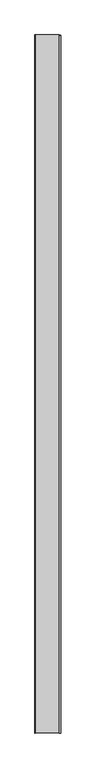
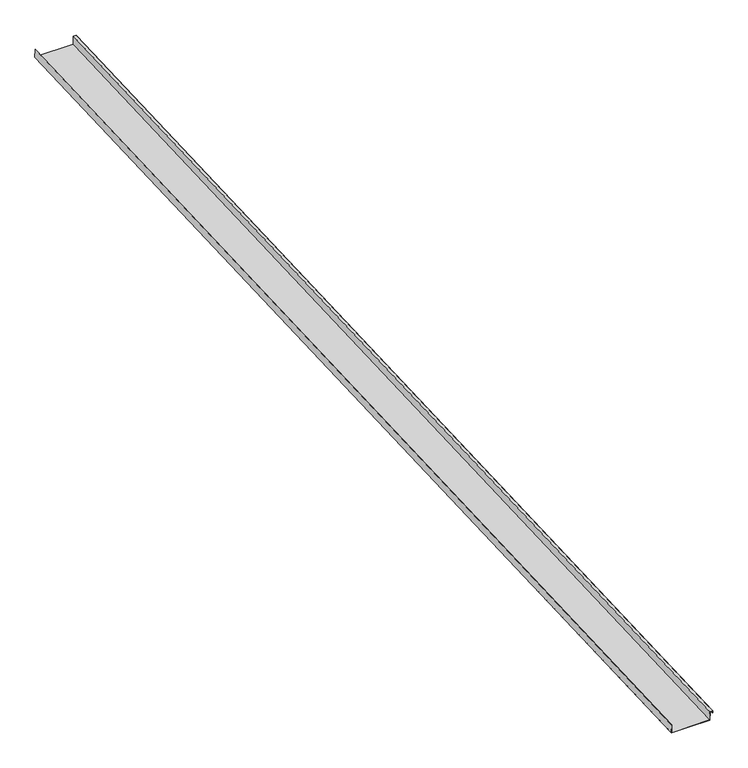
"""IFC4 building model written with IfcOpenShell, lengths in millimetres: proxy geometry, Generic Models 2:Generic Models 2:310765:Generic Models 2:310765 : Generic Models 2:Generic Models 2:310765:201 : Generic Models 2:Generic Models 2:310765:Generic Models 2:310765 : Generic Models 2:Generic Models 2:310765:300385."""

from ifc_helpers import new_model, si_unit, origin, place, context, project, spatial, faceted_brep, source, transform, mapped, element, save


def generic_models_1951ae82(model_context):
    return source(origin(), model_context, "Body", "Brep", [
        faceted_brep([(579576.913564, -579058.2473171, 4008.1996185), (579578.4218144, -579058.2473171, 4008.1996185), (579591.201064, -579058.2473171, 4008.1996185), (579591.201064, -579057.8507862, 3998.6828759), (579592.788564, -579057.8507862, 3998.6828759), (579592.788564, -579058.3134056, 4009.7857422), (579576.8343144, -579058.3134056, 4009.7857422), (579575.326064, -579058.3134056, 4009.7857422), (579575.326064, -579056.1985739, 3959.0297821), (579356.251064, -579056.1985739, 3959.0297821), (579356.251064, -579058.1812286, 4006.6134947), (579354.663564, -579058.1812286, 4006.6134947), (579354.663564, -579056.1324855, 3957.4436583), (579576.913564, -579056.1324855, 3957.4436583), (579576.913564, -572685.3337089, 4273.7376855), (579576.913564, -572683.2188772, 4222.9817254), (579354.663564, -572683.2188772, 4222.9817254), (579354.663564, -572685.2676204, 4272.1515617), (579356.251064, -572685.2676204, 4272.1515617), (579356.251064, -572683.2849657, 4224.5678491), (579575.326064, -572683.2849657, 4224.5678491), (579575.326064, -572685.3997974, 4275.3238092), (579592.788564, -572685.3997974, 4275.3238092), (579592.788564, -572684.9371779, 4264.2209429), (579591.201064, -572684.9371779, 4264.2209429), (579591.201064, -572685.3337089, 4273.7376855)], [[[0, 1, 2, 3, 4, 5, 6, 7, 8, 9, 10, 11, 12, 13]], [[14, 15, 16, 17, 18, 19, 20, 21, 22, 23, 24, 25]], [[14, 25, 2, 1, 0]], [[25, 24, 3, 2]], [[24, 23, 4, 3]], [[23, 22, 5, 4]], [[22, 21, 7, 6, 5]], [[21, 20, 8, 7]], [[20, 19, 9, 8]], [[19, 18, 10, 9]], [[18, 17, 11, 10]], [[17, 16, 12, 11]], [[16, 15, 13, 12]], [[15, 14, 0, 13]]]),
    ])


if __name__ == "__main__":
    model = new_model("IFC4")
    model_context = context("Model", 3, world=origin())
    ifc_project = project(units=[si_unit("LENGTHUNIT", "METRE", prefix="MILLI")], contexts=[model_context])
    site = spatial("IfcSite", under=ifc_project)
    building = spatial("IfcBuilding", under=site)
    placement = place(None, origin())
    generic_models_shape = generic_models_1951ae82(model_context)
    element("IfcBuildingElementProxy", 1, Name="Generic Models 2:Generic Models 2:310765:Generic Models 2:310765 : Generic Models 2:Generic Models 2:310765:201 : Generic Models 2:Generic Models 2:310765:Generic Models 2:310765 : Generic Models 2:Generic Models 2:310765:300385", ObjectType="Generic Models 2:Generic Models 2:310765:Generic Models 2:310765 : Generic Models 2:Generic Models 2:310765:201 : Generic Models 2:Generic Models 2:310765:Generic Models 2:310765 : Generic Models 2:Generic Models 2:310765:300385", at=placement, inside=building, context=model_context, shape_type="MappedRepresentation", body=[
        mapped(generic_models_shape, transform((0.0, 0.0, 0.0), x_axis=(1.0, 0.0, 0.0), y_axis=(0.0, 1.0, 0.0), z_axis=(0.0, 0.0, 1.0))),
    ])
    save(model, "model.ifc")

# Revit data of these elements
# Type "Generic Models 2:Generic Models 2:310765:Generic Models 2:310765 : Generic Models 2:Generic Models 2:310765:201 : Generic Models 2:Generic Models 2:310765:Generic Models 2:310765 : Generic Models 2:Generic Models 2:310765:300385"
#   NameOverride = "Generic Models 2:Generic Models 2:310765:Generic Models 2:310765 : Generic Models 2:Generic Models 2:310765:300385"
#   ObjectTypeOverride = "Generic Models 2:310765 : Generic Models 2:Generic Models 2:310765"
#   Reference = "Generic Models 2"
#   Tag = "300385"
# Element 1 (IfcBuildingElementProxy, "Generic Models 2:Generic Models 2:310765:Generic Models 2:310765 : Generic Models 2:Generic Models 2:310765:201 : Generic Models 2:Generic Models 2:310765:Generic Models 2:310765 : Generic Models 2:Generic Models 2:310765:300385")
#   Materials on its faces: "STRUCTURAL STANDING SEAM SHEET METAL ROOFING - BATTENLOK - COLOR T.B.D."
# Materials
#   "STRUCTURAL STANDING SEAM SHEET METAL ROOFING - BATTENLOK - COLOR T.B.D.": class "Generic", colour RGB 120 120 120, transparency 0, Cost = 0
